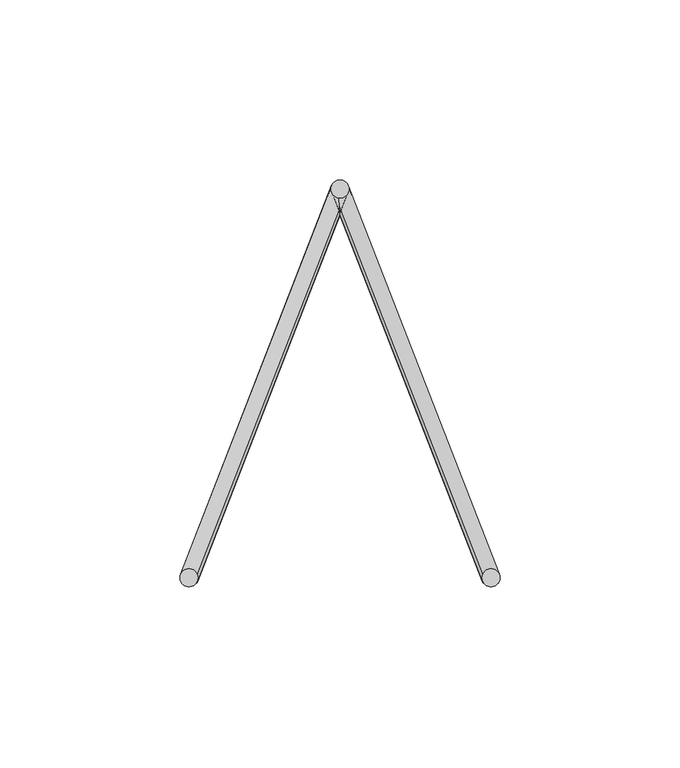
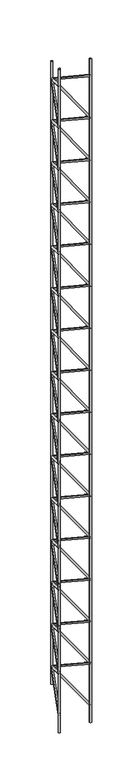
"""IFC4 building model written with IfcOpenShell, lengths in millimetres: proxy geometry, Pre-fab. (Vigota 1 - Pano 8)."""

from ifc_helpers import new_model, si_unit, point, frame, frame_2d, origin, origin_with_axes, origin_2d, place, context, project, spatial, circle_curve, trimmed, segment, composite_curve, outline, extrude, source, transform, mapped, element, save


def structural_framing_f61d2ecd(model_context):
    return source(origin(), model_context, "Body", "SweptSolid", [
        extrude(outline(composite_curve([segment(trimmed(circle_curve(origin_2d(), 2.5), [point((2.5, 0.0))], [point((-2.5, 0.0))], False, "CARTESIAN"), True, "CONTINUOUS"), segment(trimmed(circle_curve(origin_2d(), 2.5), [point((-2.5, 0.0))], [point((2.5, 0.0))], False, "CARTESIAN"), True, "CONTINUOUS")], self_intersect=False)), origin_with_axes(), (0.0, 0.0, 1.0), 1896.601886),
        extrude(outline(composite_curve([segment(trimmed(circle_curve(frame_2d((-42.0, 108.0)), 2.5), [point((-39.5, 108.0))], [point((-44.5, 108.0))], False, "CARTESIAN"), True, "CONTINUOUS"), segment(trimmed(circle_curve(frame_2d((-42.0, 108.0)), 2.5), [point((-44.5, 108.0))], [point((-39.5, 108.0))], False, "CARTESIAN"), True, "CONTINUOUS")], self_intersect=False)), frame((0.0, 0.0, 58.300943), z_axis=(0.0, 0.0, 1.0), x_axis=(1.0, 0.0, 0.0)), (0.0, 0.0, 1.0), 1780.0),
        extrude(outline(composite_curve([segment(trimmed(circle_curve(origin_2d(), 2.5), [point((2.5, 0.0))], [point((-2.5, 0.0))], False, "CARTESIAN"), True, "CONTINUOUS"), segment(trimmed(circle_curve(origin_2d(), 2.5), [point((-2.5, 0.0))], [point((2.5, 0.0))], False, "CARTESIAN"), True, "CONTINUOUS")], self_intersect=False)), frame((0.0, 0.0, 48.300943), z_axis=(-0.3218603428886276, 0.8276408817707567, 0.4598004898837537), x_axis=(0.8192319205108605, -3.936835275445103e-11, 0.5734623443750141)), (0.0, 0.0, 1.0), 130.491379),
        extrude(outline(composite_curve([segment(trimmed(circle_curve(origin_2d(), 2.5), [point((2.5, 0.0))], [point((-2.5, 0.0))], False, "CARTESIAN"), True, "CONTINUOUS"), segment(trimmed(circle_curve(origin_2d(), 2.5), [point((-2.5, 0.0))], [point((2.5, 0.0))], False, "CARTESIAN"), True, "CONTINUOUS")], self_intersect=False)), frame((-42.0, 108.0, 108.300943), z_axis=(0.3218603428886276, -0.8276408817707567, 0.4598004898837537), x_axis=(0.8192319205108605, -3.936835275445103e-11, -0.5734623443750141)), (0.0, 0.0, 1.0), 130.491379),
        extrude(outline(composite_curve([segment(trimmed(circle_curve(origin_2d(), 2.5), [point((2.5, 0.0))], [point((-2.5, 0.0))], False, "CARTESIAN"), True, "CONTINUOUS"), segment(trimmed(circle_curve(origin_2d(), 2.5), [point((-2.5, 0.0))], [point((2.5, 0.0))], False, "CARTESIAN"), True, "CONTINUOUS")], self_intersect=False)), frame((0.0, 0.0, 168.300943), z_axis=(-0.3218603428886276, 0.8276408817707567, 0.4598004898837537), x_axis=(0.8192319205108605, -3.936835275445103e-11, 0.5734623443750141)), (0.0, 0.0, 1.0), 130.491379),
        extrude(outline(composite_curve([segment(trimmed(circle_curve(origin_2d(), 2.5), [point((2.5, 0.0))], [point((-2.5, 0.0))], False, "CARTESIAN"), True, "CONTINUOUS"), segment(trimmed(circle_curve(origin_2d(), 2.5), [point((-2.5, 0.0))], [point((2.5, 0.0))], False, "CARTESIAN"), True, "CONTINUOUS")], self_intersect=False)), frame((-42.0, 108.0, 228.300943), z_axis=(0.3218603428886276, -0.8276408817707567, 0.4598004898837537), x_axis=(0.8192319205108605, -3.936835275445103e-11, -0.5734623443750141)), (0.0, 0.0, 1.0), 130.491379),
        extrude(outline(composite_curve([segment(trimmed(circle_curve(origin_2d(), 2.5), [point((2.5, 0.0))], [point((-2.5, 0.0))], False, "CARTESIAN"), True, "CONTINUOUS"), segment(trimmed(circle_curve(origin_2d(), 2.5), [point((-2.5, 0.0))], [point((2.5, 0.0))], False, "CARTESIAN"), True, "CONTINUOUS")], self_intersect=False)), frame((0.0, 0.0, 288.300943), z_axis=(-0.3218603428886276, 0.8276408817707567, 0.4598004898837537), x_axis=(0.8192319205108605, -3.936835275445103e-11, 0.5734623443750141)), (0.0, 0.0, 1.0), 130.491379),
        extrude(outline(composite_curve([segment(trimmed(circle_curve(origin_2d(), 2.5), [point((2.5, 0.0))], [point((-2.5, 0.0))], False, "CARTESIAN"), True, "CONTINUOUS"), segment(trimmed(circle_curve(origin_2d(), 2.5), [point((-2.5, 0.0))], [point((2.5, 0.0))], False, "CARTESIAN"), True, "CONTINUOUS")], self_intersect=False)), frame((-42.0, 108.0, 348.300943), z_axis=(0.3218603428886276, -0.8276408817707567, 0.4598004898837537), x_axis=(0.8192319205108605, -3.936835275445103e-11, -0.5734623443750141)), (0.0, 0.0, 1.0), 130.491379),
        extrude(outline(composite_curve([segment(trimmed(circle_curve(origin_2d(), 2.5), [point((2.5, 0.0))], [point((-2.5, 0.0))], False, "CARTESIAN"), True, "CONTINUOUS"), segment(trimmed(circle_curve(origin_2d(), 2.5), [point((-2.5, 0.0))], [point((2.5, 0.0))], False, "CARTESIAN"), True, "CONTINUOUS")], self_intersect=False)), frame((0.0, 0.0, 408.300943), z_axis=(-0.3218603428886276, 0.8276408817707567, 0.4598004898837537), x_axis=(0.8192319205108605, -3.936835275445103e-11, 0.5734623443750141)), (0.0, 0.0, 1.0), 130.491379),
        extrude(outline(composite_curve([segment(trimmed(circle_curve(origin_2d(), 2.5), [point((2.5, 0.0))], [point((-2.5, 0.0))], False, "CARTESIAN"), True, "CONTINUOUS"), segment(trimmed(circle_curve(origin_2d(), 2.5), [point((-2.5, 0.0))], [point((2.5, 0.0))], False, "CARTESIAN"), True, "CONTINUOUS")], self_intersect=False)), frame((-42.0, 108.0, 468.300943), z_axis=(0.3218603428886276, -0.8276408817707567, 0.4598004898837537), x_axis=(0.8192319205108605, -3.936835275445103e-11, -0.5734623443750141)), (0.0, 0.0, 1.0), 130.491379),
        extrude(outline(composite_curve([segment(trimmed(circle_curve(origin_2d(), 2.5), [point((2.5, 0.0))], [point((-2.5, 0.0))], False, "CARTESIAN"), True, "CONTINUOUS"), segment(trimmed(circle_curve(origin_2d(), 2.5), [point((-2.5, 0.0))], [point((2.5, 0.0))], False, "CARTESIAN"), True, "CONTINUOUS")], self_intersect=False)), frame((0.0, 0.0, 528.300943), z_axis=(-0.3218603428886276, 0.8276408817707567, 0.4598004898837537), x_axis=(0.8192319205108605, -3.936835275445103e-11, 0.5734623443750141)), (0.0, 0.0, 1.0), 130.491379),
        extrude(outline(composite_curve([segment(trimmed(circle_curve(origin_2d(), 2.5), [point((2.5, 0.0))], [point((-2.5, 0.0))], False, "CARTESIAN"), True, "CONTINUOUS"), segment(trimmed(circle_curve(origin_2d(), 2.5), [point((-2.5, 0.0))], [point((2.5, 0.0))], False, "CARTESIAN"), True, "CONTINUOUS")], self_intersect=False)), frame((-42.0, 108.0, 588.300943), z_axis=(0.3218603428886276, -0.8276408817707567, 0.4598004898837537), x_axis=(0.8192319205108605, -3.936835275445103e-11, -0.5734623443750141)), (0.0, 0.0, 1.0), 130.491379),
        extrude(outline(composite_curve([segment(trimmed(circle_curve(origin_2d(), 2.5), [point((2.5, 0.0))], [point((-2.5, 0.0))], False, "CARTESIAN"), True, "CONTINUOUS"), segment(trimmed(circle_curve(origin_2d(), 2.5), [point((-2.5, 0.0))], [point((2.5, 0.0))], False, "CARTESIAN"), True, "CONTINUOUS")], self_intersect=False)), frame((0.0, 0.0, 648.300943), z_axis=(-0.3218603428886276, 0.8276408817707567, 0.4598004898837537), x_axis=(0.8192319205108605, -3.936835275445103e-11, 0.5734623443750141)), (0.0, 0.0, 1.0), 130.491379),
        extrude(outline(composite_curve([segment(trimmed(circle_curve(origin_2d(), 2.5), [point((2.5, 0.0))], [point((-2.5, 0.0))], False, "CARTESIAN"), True, "CONTINUOUS"), segment(trimmed(circle_curve(origin_2d(), 2.5), [point((-2.5, 0.0))], [point((2.5, 0.0))], False, "CARTESIAN"), True, "CONTINUOUS")], self_intersect=False)), frame((-42.0, 108.0, 708.300943), z_axis=(0.3218603428886276, -0.8276408817707567, 0.4598004898837537), x_axis=(0.8192319205108605, -3.936835275445103e-11, -0.5734623443750141)), (0.0, 0.0, 1.0), 130.491379),
        extrude(outline(composite_curve([segment(trimmed(circle_curve(origin_2d(), 2.5), [point((2.5, 0.0))], [point((-2.5, 0.0))], False, "CARTESIAN"), True, "CONTINUOUS"), segment(trimmed(circle_curve(origin_2d(), 2.5), [point((-2.5, 0.0))], [point((2.5, 0.0))], False, "CARTESIAN"), True, "CONTINUOUS")], self_intersect=False)), frame((0.0, 0.0, 768.300943), z_axis=(-0.3218603428886276, 0.8276408817707567, 0.4598004898837537), x_axis=(0.8192319205108605, -3.936835275445103e-11, 0.5734623443750141)), (0.0, 0.0, 1.0), 130.491379),
        extrude(outline(composite_curve([segment(trimmed(circle_curve(origin_2d(), 2.5), [point((2.5, 0.0))], [point((-2.5, 0.0))], False, "CARTESIAN"), True, "CONTINUOUS"), segment(trimmed(circle_curve(origin_2d(), 2.5), [point((-2.5, 0.0))], [point((2.5, 0.0))], False, "CARTESIAN"), True, "CONTINUOUS")], self_intersect=False)), frame((-42.0, 108.0, 828.300943), z_axis=(0.3218603428886276, -0.8276408817707567, 0.4598004898837537), x_axis=(0.8192319205108605, -3.936835275445103e-11, -0.5734623443750141)), (0.0, 0.0, 1.0), 130.491379),
        extrude(outline(composite_curve([segment(trimmed(circle_curve(origin_2d(), 2.5), [point((2.5, 0.0))], [point((-2.5, 0.0))], False, "CARTESIAN"), True, "CONTINUOUS"), segment(trimmed(circle_curve(origin_2d(), 2.5), [point((-2.5, 0.0))], [point((2.5, 0.0))], False, "CARTESIAN"), True, "CONTINUOUS")], self_intersect=False)), frame((0.0, 0.0, 888.300943), z_axis=(-0.3218603428886276, 0.8276408817707567, 0.4598004898837537), x_axis=(0.8192319205108605, -3.936835275445103e-11, 0.5734623443750141)), (0.0, 0.0, 1.0), 130.491379),
        extrude(outline(composite_curve([segment(trimmed(circle_curve(origin_2d(), 2.5), [point((2.5, 0.0))], [point((-2.5, 0.0))], False, "CARTESIAN"), True, "CONTINUOUS"), segment(trimmed(circle_curve(origin_2d(), 2.5), [point((-2.5, 0.0))], [point((2.5, 0.0))], False, "CARTESIAN"), True, "CONTINUOUS")], self_intersect=False)), frame((-42.0, 108.0, 948.300943), z_axis=(0.3218603428886276, -0.8276408817707567, 0.4598004898837537), x_axis=(0.8192319205108605, -3.936835275445103e-11, -0.5734623443750141)), (0.0, 0.0, 1.0), 130.491379),
        extrude(outline(composite_curve([segment(trimmed(circle_curve(origin_2d(), 2.5), [point((2.5, 0.0))], [point((-2.5, 0.0))], False, "CARTESIAN"), True, "CONTINUOUS"), segment(trimmed(circle_curve(origin_2d(), 2.5), [point((-2.5, 0.0))], [point((2.5, 0.0))], False, "CARTESIAN"), True, "CONTINUOUS")], self_intersect=False)), frame((0.0, 0.0, 1008.300943), z_axis=(-0.3218603428886276, 0.8276408817707567, 0.4598004898837537), x_axis=(0.8192319205108605, -3.936835275445103e-11, 0.5734623443750141)), (0.0, 0.0, 1.0), 130.491379),
        extrude(outline(composite_curve([segment(trimmed(circle_curve(origin_2d(), 2.5), [point((2.5, 0.0))], [point((-2.5, 0.0))], False, "CARTESIAN"), True, "CONTINUOUS"), segment(trimmed(circle_curve(origin_2d(), 2.5), [point((-2.5, 0.0))], [point((2.5, 0.0))], False, "CARTESIAN"), True, "CONTINUOUS")], self_intersect=False)), frame((-42.0, 108.0, 1068.300943), z_axis=(0.3218603428886276, -0.8276408817707567, 0.4598004898837537), x_axis=(0.8192319205108605, -3.936835275445103e-11, -0.5734623443750141)), (0.0, 0.0, 1.0), 130.491379),
        extrude(outline(composite_curve([segment(trimmed(circle_curve(origin_2d(), 2.5), [point((2.5, 0.0))], [point((-2.5, 0.0))], False, "CARTESIAN"), True, "CONTINUOUS"), segment(trimmed(circle_curve(origin_2d(), 2.5), [point((-2.5, 0.0))], [point((2.5, 0.0))], False, "CARTESIAN"), True, "CONTINUOUS")], self_intersect=False)), frame((0.0, 0.0, 1128.300943), z_axis=(-0.3218603428886276, 0.8276408817707567, 0.4598004898837537), x_axis=(0.8192319205108605, -3.936835275445103e-11, 0.5734623443750141)), (0.0, 0.0, 1.0), 130.491379),
        extrude(outline(composite_curve([segment(trimmed(circle_curve(origin_2d(), 2.5), [point((2.5, 0.0))], [point((-2.5, 0.0))], False, "CARTESIAN"), True, "CONTINUOUS"), segment(trimmed(circle_curve(origin_2d(), 2.5), [point((-2.5, 0.0))], [point((2.5, 0.0))], False, "CARTESIAN"), True, "CONTINUOUS")], self_intersect=False)), frame((-42.0, 108.0, 1188.300943), z_axis=(0.3218603428886276, -0.8276408817707567, 0.4598004898837537), x_axis=(0.8192319205108605, -3.936835275445103e-11, -0.5734623443750141)), (0.0, 0.0, 1.0), 130.491379),
        extrude(outline(composite_curve([segment(trimmed(circle_curve(origin_2d(), 2.5), [point((2.5, 0.0))], [point((-2.5, 0.0))], False, "CARTESIAN"), True, "CONTINUOUS"), segment(trimmed(circle_curve(origin_2d(), 2.5), [point((-2.5, 0.0))], [point((2.5, 0.0))], False, "CARTESIAN"), True, "CONTINUOUS")], self_intersect=False)), frame((0.0, 0.0, 1248.300943), z_axis=(-0.3218603428886276, 0.8276408817707567, 0.4598004898837537), x_axis=(0.8192319205108605, -3.936835275445103e-11, 0.5734623443750141)), (0.0, 0.0, 1.0), 130.491379),
        extrude(outline(composite_curve([segment(trimmed(circle_curve(origin_2d(), 2.5), [point((2.5, 0.0))], [point((-2.5, 0.0))], False, "CARTESIAN"), True, "CONTINUOUS"), segment(trimmed(circle_curve(origin_2d(), 2.5), [point((-2.5, 0.0))], [point((2.5, 0.0))], False, "CARTESIAN"), True, "CONTINUOUS")], self_intersect=False)), frame((-42.0, 108.0, 1308.300943), z_axis=(0.3218603428886276, -0.8276408817707567, 0.4598004898837537), x_axis=(0.8192319205108605, -3.936835275445103e-11, -0.5734623443750141)), (0.0, 0.0, 1.0), 130.491379),
        extrude(outline(composite_curve([segment(trimmed(circle_curve(origin_2d(), 2.5), [point((2.5, 0.0))], [point((-2.5, 0.0))], False, "CARTESIAN"), True, "CONTINUOUS"), segment(trimmed(circle_curve(origin_2d(), 2.5), [point((-2.5, 0.0))], [point((2.5, 0.0))], False, "CARTESIAN"), True, "CONTINUOUS")], self_intersect=False)), frame((0.0, 0.0, 1368.300943), z_axis=(-0.3218603428886276, 0.8276408817707567, 0.4598004898837537), x_axis=(0.8192319205108605, -3.936835275445103e-11, 0.5734623443750141)), (0.0, 0.0, 1.0), 130.491379),
        extrude(outline(composite_curve([segment(trimmed(circle_curve(origin_2d(), 2.5), [point((2.5, 0.0))], [point((-2.5, 0.0))], False, "CARTESIAN"), True, "CONTINUOUS"), segment(trimmed(circle_curve(origin_2d(), 2.5), [point((-2.5, 0.0))], [point((2.5, 0.0))], False, "CARTESIAN"), True, "CONTINUOUS")], self_intersect=False)), frame((-42.0, 108.0, 1428.300943), z_axis=(0.3218603428886276, -0.8276408817707567, 0.4598004898837537), x_axis=(0.8192319205108605, -3.936835275445103e-11, -0.5734623443750141)), (0.0, 0.0, 1.0), 130.491379),
        extrude(outline(composite_curve([segment(trimmed(circle_curve(origin_2d(), 2.5), [point((2.5, 0.0))], [point((-2.5, 0.0))], False, "CARTESIAN"), True, "CONTINUOUS"), segment(trimmed(circle_curve(origin_2d(), 2.5), [point((-2.5, 0.0))], [point((2.5, 0.0))], False, "CARTESIAN"), True, "CONTINUOUS")], self_intersect=False)), frame((0.0, 0.0, 1488.300943), z_axis=(-0.3218603428886276, 0.8276408817707567, 0.4598004898837537), x_axis=(0.8192319205108605, -3.936835275445103e-11, 0.5734623443750141)), (0.0, 0.0, 1.0), 130.491379),
        extrude(outline(composite_curve([segment(trimmed(circle_curve(origin_2d(), 2.5), [point((2.5, 0.0))], [point((-2.5, 0.0))], False, "CARTESIAN"), True, "CONTINUOUS"), segment(trimmed(circle_curve(origin_2d(), 2.5), [point((-2.5, 0.0))], [point((2.5, 0.0))], False, "CARTESIAN"), True, "CONTINUOUS")], self_intersect=False)), frame((-42.0, 108.0, 1548.300943), z_axis=(0.3218603428886276, -0.8276408817707567, 0.4598004898837537), x_axis=(0.8192319205108605, -3.936835275445103e-11, -0.5734623443750141)), (0.0, 0.0, 1.0), 130.491379),
        extrude(outline(composite_curve([segment(trimmed(circle_curve(origin_2d(), 2.5), [point((2.5, 0.0))], [point((-2.5, 0.0))], False, "CARTESIAN"), True, "CONTINUOUS"), segment(trimmed(circle_curve(origin_2d(), 2.5), [point((-2.5, 0.0))], [point((2.5, 0.0))], False, "CARTESIAN"), True, "CONTINUOUS")], self_intersect=False)), frame((0.0, 0.0, 1608.300943), z_axis=(-0.3218603428886276, 0.8276408817707567, 0.4598004898837537), x_axis=(0.8192319205108605, -3.936835275445103e-11, 0.5734623443750141)), (0.0, 0.0, 1.0), 130.491379),
        extrude(outline(composite_curve([segment(trimmed(circle_curve(origin_2d(), 2.5), [point((2.5, 0.0))], [point((-2.5, 0.0))], False, "CARTESIAN"), True, "CONTINUOUS"), segment(trimmed(circle_curve(origin_2d(), 2.5), [point((-2.5, 0.0))], [point((2.5, 0.0))], False, "CARTESIAN"), True, "CONTINUOUS")], self_intersect=False)), frame((-42.0, 108.0, 1668.300943), z_axis=(0.3218603428886276, -0.8276408817707567, 0.4598004898837537), x_axis=(0.8192319205108605, -3.936835275445103e-11, -0.5734623443750141)), (0.0, 0.0, 1.0), 130.491379),
        extrude(outline(composite_curve([segment(trimmed(circle_curve(origin_2d(), 2.5), [point((2.5, 0.0))], [point((-2.5, 0.0))], False, "CARTESIAN"), True, "CONTINUOUS"), segment(trimmed(circle_curve(origin_2d(), 2.5), [point((-2.5, 0.0))], [point((2.5, 0.0))], False, "CARTESIAN"), True, "CONTINUOUS")], self_intersect=False)), frame((0.0, 0.0, 1728.300943), z_axis=(-0.3218603428886276, 0.8276408817707567, 0.4598004898837537), x_axis=(0.8192319205108605, -3.936835275445103e-11, 0.5734623443750141)), (0.0, 0.0, 1.0), 130.491379),
        extrude(outline(composite_curve([segment(trimmed(circle_curve(origin_2d(), 2.5), [point((2.5, 0.0))], [point((-2.5, 0.0))], False, "CARTESIAN"), True, "CONTINUOUS"), segment(trimmed(circle_curve(origin_2d(), 2.5), [point((-2.5, 0.0))], [point((2.5, 0.0))], False, "CARTESIAN"), True, "CONTINUOUS")], self_intersect=False)), frame((-42.0, 108.0, 1788.300943), z_axis=(0.3218603428886276, -0.8276408817707567, 0.4598004898837537), x_axis=(0.8192319205108605, -3.936835275445103e-11, -0.5734623443750141)), (0.0, 0.0, 1.0), 130.491379),
        extrude(outline(composite_curve([segment(trimmed(circle_curve(frame_2d((-84.0, 0.0)), 2.5), [point((-81.5, 0.0))], [point((-86.5, 0.0))], False, "CARTESIAN"), True, "CONTINUOUS"), segment(trimmed(circle_curve(frame_2d((-84.0, 0.0)), 2.5), [point((-86.5, 0.0))], [point((-81.5, 0.0))], False, "CARTESIAN"), True, "CONTINUOUS")], self_intersect=False)), origin_with_axes(), (0.0, 0.0, 1.0), 1896.601886),
        extrude(outline(composite_curve([segment(trimmed(circle_curve(origin_2d(), 2.5), [point((2.5, 0.0))], [point((-2.5, 0.0))], False, "CARTESIAN"), True, "CONTINUOUS"), segment(trimmed(circle_curve(origin_2d(), 2.5), [point((-2.5, 0.0))], [point((2.5, 0.0))], False, "CARTESIAN"), True, "CONTINUOUS")], self_intersect=False)), frame((-84.0, 0.0, 48.300943), z_axis=(0.3218603428886276, 0.8276408817707567, 0.4598004898837537), x_axis=(0.8192319205108605, 3.936835275445103e-11, -0.5734623443750141)), (0.0, 0.0, 1.0), 130.491379),
        extrude(outline(composite_curve([segment(trimmed(circle_curve(origin_2d(), 2.5), [point((2.5, 0.0))], [point((-2.5, 0.0))], False, "CARTESIAN"), True, "CONTINUOUS"), segment(trimmed(circle_curve(origin_2d(), 2.5), [point((-2.5, 0.0))], [point((2.5, 0.0))], False, "CARTESIAN"), True, "CONTINUOUS")], self_intersect=False)), frame((-42.0, 108.0, 108.300943), z_axis=(-0.3218603428886276, -0.8276408817707567, 0.4598004898837537), x_axis=(0.8192319205108605, 3.936835275445103e-11, 0.5734623443750141)), (0.0, 0.0, 1.0), 130.491379),
        extrude(outline(composite_curve([segment(trimmed(circle_curve(origin_2d(), 2.5), [point((2.5, 0.0))], [point((-2.5, 0.0))], False, "CARTESIAN"), True, "CONTINUOUS"), segment(trimmed(circle_curve(origin_2d(), 2.5), [point((-2.5, 0.0))], [point((2.5, 0.0))], False, "CARTESIAN"), True, "CONTINUOUS")], self_intersect=False)), frame((-84.0, 0.0, 168.300943), z_axis=(0.3218603428886276, 0.8276408817707567, 0.4598004898837537), x_axis=(0.8192319205108605, 3.936835275445103e-11, -0.5734623443750141)), (0.0, 0.0, 1.0), 130.491379),
        extrude(outline(composite_curve([segment(trimmed(circle_curve(origin_2d(), 2.5), [point((2.5, 0.0))], [point((-2.5, 0.0))], False, "CARTESIAN"), True, "CONTINUOUS"), segment(trimmed(circle_curve(origin_2d(), 2.5), [point((-2.5, 0.0))], [point((2.5, 0.0))], False, "CARTESIAN"), True, "CONTINUOUS")], self_intersect=False)), frame((-42.0, 108.0, 228.300943), z_axis=(-0.3218603428886276, -0.8276408817707567, 0.4598004898837537), x_axis=(0.8192319205108605, 3.936835275445103e-11, 0.5734623443750141)), (0.0, 0.0, 1.0), 130.491379),
        extrude(outline(composite_curve([segment(trimmed(circle_curve(origin_2d(), 2.5), [point((2.5, 0.0))], [point((-2.5, 0.0))], False, "CARTESIAN"), True, "CONTINUOUS"), segment(trimmed(circle_curve(origin_2d(), 2.5), [point((-2.5, 0.0))], [point((2.5, 0.0))], False, "CARTESIAN"), True, "CONTINUOUS")], self_intersect=False)), frame((-84.0, 0.0, 288.300943), z_axis=(0.3218603428886276, 0.8276408817707567, 0.4598004898837537), x_axis=(0.8192319205108605, 3.936835275445103e-11, -0.5734623443750141)), (0.0, 0.0, 1.0), 130.491379),
        extrude(outline(composite_curve([segment(trimmed(circle_curve(origin_2d(), 2.5), [point((2.5, 0.0))], [point((-2.5, 0.0))], False, "CARTESIAN"), True, "CONTINUOUS"), segment(trimmed(circle_curve(origin_2d(), 2.5), [point((-2.5, 0.0))], [point((2.5, 0.0))], False, "CARTESIAN"), True, "CONTINUOUS")], self_intersect=False)), frame((-42.0, 108.0, 348.300943), z_axis=(-0.3218603428886276, -0.8276408817707567, 0.4598004898837537), x_axis=(0.8192319205108605, 3.936835275445103e-11, 0.5734623443750141)), (0.0, 0.0, 1.0), 130.491379),
        extrude(outline(composite_curve([segment(trimmed(circle_curve(origin_2d(), 2.5), [point((2.5, 0.0))], [point((-2.5, 0.0))], False, "CARTESIAN"), True, "CONTINUOUS"), segment(trimmed(circle_curve(origin_2d(), 2.5), [point((-2.5, 0.0))], [point((2.5, 0.0))], False, "CARTESIAN"), True, "CONTINUOUS")], self_intersect=False)), frame((-84.0, 0.0, 408.300943), z_axis=(0.3218603428886276, 0.8276408817707567, 0.4598004898837537), x_axis=(0.8192319205108605, 3.936835275445103e-11, -0.5734623443750141)), (0.0, 0.0, 1.0), 130.491379),
        extrude(outline(composite_curve([segment(trimmed(circle_curve(origin_2d(), 2.5), [point((2.5, 0.0))], [point((-2.5, 0.0))], False, "CARTESIAN"), True, "CONTINUOUS"), segment(trimmed(circle_curve(origin_2d(), 2.5), [point((-2.5, 0.0))], [point((2.5, 0.0))], False, "CARTESIAN"), True, "CONTINUOUS")], self_intersect=False)), frame((-42.0, 108.0, 468.300943), z_axis=(-0.3218603428886276, -0.8276408817707567, 0.4598004898837537), x_axis=(0.8192319205108605, 3.936835275445103e-11, 0.5734623443750141)), (0.0, 0.0, 1.0), 130.491379),
        extrude(outline(composite_curve([segment(trimmed(circle_curve(origin_2d(), 2.5), [point((2.5, 0.0))], [point((-2.5, 0.0))], False, "CARTESIAN"), True, "CONTINUOUS"), segment(trimmed(circle_curve(origin_2d(), 2.5), [point((-2.5, 0.0))], [point((2.5, 0.0))], False, "CARTESIAN"), True, "CONTINUOUS")], self_intersect=False)), frame((-84.0, 0.0, 528.300943), z_axis=(0.3218603428886276, 0.8276408817707567, 0.4598004898837537), x_axis=(0.8192319205108605, 3.936835275445103e-11, -0.5734623443750141)), (0.0, 0.0, 1.0), 130.491379),
        extrude(outline(composite_curve([segment(trimmed(circle_curve(origin_2d(), 2.5), [point((2.5, 0.0))], [point((-2.5, 0.0))], False, "CARTESIAN"), True, "CONTINUOUS"), segment(trimmed(circle_curve(origin_2d(), 2.5), [point((-2.5, 0.0))], [point((2.5, 0.0))], False, "CARTESIAN"), True, "CONTINUOUS")], self_intersect=False)), frame((-42.0, 108.0, 588.300943), z_axis=(-0.3218603428886276, -0.8276408817707567, 0.4598004898837537), x_axis=(0.8192319205108605, 3.936835275445103e-11, 0.5734623443750141)), (0.0, 0.0, 1.0), 130.491379),
        extrude(outline(composite_curve([segment(trimmed(circle_curve(origin_2d(), 2.5), [point((2.5, 0.0))], [point((-2.5, 0.0))], False, "CARTESIAN"), True, "CONTINUOUS"), segment(trimmed(circle_curve(origin_2d(), 2.5), [point((-2.5, 0.0))], [point((2.5, 0.0))], False, "CARTESIAN"), True, "CONTINUOUS")], self_intersect=False)), frame((-84.0, 0.0, 648.300943), z_axis=(0.3218603428886276, 0.8276408817707567, 0.4598004898837537), x_axis=(0.8192319205108605, 3.936835275445103e-11, -0.5734623443750141)), (0.0, 0.0, 1.0), 130.491379),
        extrude(outline(composite_curve([segment(trimmed(circle_curve(origin_2d(), 2.5), [point((2.5, 0.0))], [point((-2.5, 0.0))], False, "CARTESIAN"), True, "CONTINUOUS"), segment(trimmed(circle_curve(origin_2d(), 2.5), [point((-2.5, 0.0))], [point((2.5, 0.0))], False, "CARTESIAN"), True, "CONTINUOUS")], self_intersect=False)), frame((-42.0, 108.0, 708.300943), z_axis=(-0.3218603428886276, -0.8276408817707567, 0.4598004898837537), x_axis=(0.8192319205108605, 3.936835275445103e-11, 0.5734623443750141)), (0.0, 0.0, 1.0), 130.491379),
        extrude(outline(composite_curve([segment(trimmed(circle_curve(origin_2d(), 2.5), [point((2.5, 0.0))], [point((-2.5, 0.0))], False, "CARTESIAN"), True, "CONTINUOUS"), segment(trimmed(circle_curve(origin_2d(), 2.5), [point((-2.5, 0.0))], [point((2.5, 0.0))], False, "CARTESIAN"), True, "CONTINUOUS")], self_intersect=False)), frame((-84.0, 0.0, 768.300943), z_axis=(0.3218603428886276, 0.8276408817707567, 0.4598004898837537), x_axis=(0.8192319205108605, 3.936835275445103e-11, -0.5734623443750141)), (0.0, 0.0, 1.0), 130.491379),
        extrude(outline(composite_curve([segment(trimmed(circle_curve(origin_2d(), 2.5), [point((2.5, 0.0))], [point((-2.5, 0.0))], False, "CARTESIAN"), True, "CONTINUOUS"), segment(trimmed(circle_curve(origin_2d(), 2.5), [point((-2.5, 0.0))], [point((2.5, 0.0))], False, "CARTESIAN"), True, "CONTINUOUS")], self_intersect=False)), frame((-42.0, 108.0, 828.300943), z_axis=(-0.3218603428886276, -0.8276408817707567, 0.4598004898837537), x_axis=(0.8192319205108605, 3.936835275445103e-11, 0.5734623443750141)), (0.0, 0.0, 1.0), 130.491379),
        extrude(outline(composite_curve([segment(trimmed(circle_curve(origin_2d(), 2.5), [point((2.5, 0.0))], [point((-2.5, 0.0))], False, "CARTESIAN"), True, "CONTINUOUS"), segment(trimmed(circle_curve(origin_2d(), 2.5), [point((-2.5, 0.0))], [point((2.5, 0.0))], False, "CARTESIAN"), True, "CONTINUOUS")], self_intersect=False)), frame((-84.0, 0.0, 888.300943), z_axis=(0.3218603428886276, 0.8276408817707567, 0.4598004898837537), x_axis=(0.8192319205108605, 3.936835275445103e-11, -0.5734623443750141)), (0.0, 0.0, 1.0), 130.491379),
        extrude(outline(composite_curve([segment(trimmed(circle_curve(origin_2d(), 2.5), [point((2.5, 0.0))], [point((-2.5, 0.0))], False, "CARTESIAN"), True, "CONTINUOUS"), segment(trimmed(circle_curve(origin_2d(), 2.5), [point((-2.5, 0.0))], [point((2.5, 0.0))], False, "CARTESIAN"), True, "CONTINUOUS")], self_intersect=False)), frame((-42.0, 108.0, 948.300943), z_axis=(-0.3218603428886276, -0.8276408817707567, 0.4598004898837537), x_axis=(0.8192319205108605, 3.936835275445103e-11, 0.5734623443750141)), (0.0, 0.0, 1.0), 130.491379),
        extrude(outline(composite_curve([segment(trimmed(circle_curve(origin_2d(), 2.5), [point((2.5, 0.0))], [point((-2.5, 0.0))], False, "CARTESIAN"), True, "CONTINUOUS"), segment(trimmed(circle_curve(origin_2d(), 2.5), [point((-2.5, 0.0))], [point((2.5, 0.0))], False, "CARTESIAN"), True, "CONTINUOUS")], self_intersect=False)), frame((-84.0, 0.0, 1008.300943), z_axis=(0.3218603428886276, 0.8276408817707567, 0.4598004898837537), x_axis=(0.8192319205108605, 3.936835275445103e-11, -0.5734623443750141)), (0.0, 0.0, 1.0), 130.491379),
        extrude(outline(composite_curve([segment(trimmed(circle_curve(origin_2d(), 2.5), [point((2.5, 0.0))], [point((-2.5, 0.0))], False, "CARTESIAN"), True, "CONTINUOUS"), segment(trimmed(circle_curve(origin_2d(), 2.5), [point((-2.5, 0.0))], [point((2.5, 0.0))], False, "CARTESIAN"), True, "CONTINUOUS")], self_intersect=False)), frame((-42.0, 108.0, 1068.300943), z_axis=(-0.3218603428886276, -0.8276408817707567, 0.4598004898837537), x_axis=(0.8192319205108605, 3.936835275445103e-11, 0.5734623443750141)), (0.0, 0.0, 1.0), 130.491379),
        extrude(outline(composite_curve([segment(trimmed(circle_curve(origin_2d(), 2.5), [point((2.5, 0.0))], [point((-2.5, 0.0))], False, "CARTESIAN"), True, "CONTINUOUS"), segment(trimmed(circle_curve(origin_2d(), 2.5), [point((-2.5, 0.0))], [point((2.5, 0.0))], False, "CARTESIAN"), True, "CONTINUOUS")], self_intersect=False)), frame((-84.0, 0.0, 1128.300943), z_axis=(0.3218603428886276, 0.8276408817707567, 0.4598004898837537), x_axis=(0.8192319205108605, 3.936835275445103e-11, -0.5734623443750141)), (0.0, 0.0, 1.0), 130.491379),
        extrude(outline(composite_curve([segment(trimmed(circle_curve(origin_2d(), 2.5), [point((2.5, 0.0))], [point((-2.5, 0.0))], False, "CARTESIAN"), True, "CONTINUOUS"), segment(trimmed(circle_curve(origin_2d(), 2.5), [point((-2.5, 0.0))], [point((2.5, 0.0))], False, "CARTESIAN"), True, "CONTINUOUS")], self_intersect=False)), frame((-42.0, 108.0, 1188.300943), z_axis=(-0.3218603428886276, -0.8276408817707567, 0.4598004898837537), x_axis=(0.8192319205108605, 3.936835275445103e-11, 0.5734623443750141)), (0.0, 0.0, 1.0), 130.491379),
        extrude(outline(composite_curve([segment(trimmed(circle_curve(origin_2d(), 2.5), [point((2.5, 0.0))], [point((-2.5, 0.0))], False, "CARTESIAN"), True, "CONTINUOUS"), segment(trimmed(circle_curve(origin_2d(), 2.5), [point((-2.5, 0.0))], [point((2.5, 0.0))], False, "CARTESIAN"), True, "CONTINUOUS")], self_intersect=False)), frame((-84.0, 0.0, 1248.300943), z_axis=(0.3218603428886276, 0.8276408817707567, 0.4598004898837537), x_axis=(0.8192319205108605, 3.936835275445103e-11, -0.5734623443750141)), (0.0, 0.0, 1.0), 130.491379),
        extrude(outline(composite_curve([segment(trimmed(circle_curve(origin_2d(), 2.5), [point((2.5, 0.0))], [point((-2.5, 0.0))], False, "CARTESIAN"), True, "CONTINUOUS"), segment(trimmed(circle_curve(origin_2d(), 2.5), [point((-2.5, 0.0))], [point((2.5, 0.0))], False, "CARTESIAN"), True, "CONTINUOUS")], self_intersect=False)), frame((-42.0, 108.0, 1308.300943), z_axis=(-0.3218603428886276, -0.8276408817707567, 0.4598004898837537), x_axis=(0.8192319205108605, 3.936835275445103e-11, 0.5734623443750141)), (0.0, 0.0, 1.0), 130.491379),
        extrude(outline(composite_curve([segment(trimmed(circle_curve(origin_2d(), 2.5), [point((2.5, 0.0))], [point((-2.5, 0.0))], False, "CARTESIAN"), True, "CONTINUOUS"), segment(trimmed(circle_curve(origin_2d(), 2.5), [point((-2.5, 0.0))], [point((2.5, 0.0))], False, "CARTESIAN"), True, "CONTINUOUS")], self_intersect=False)), frame((-84.0, 0.0, 1368.300943), z_axis=(0.3218603428886276, 0.8276408817707567, 0.4598004898837537), x_axis=(0.8192319205108605, 3.936835275445103e-11, -0.5734623443750141)), (0.0, 0.0, 1.0), 130.491379),
        extrude(outline(composite_curve([segment(trimmed(circle_curve(origin_2d(), 2.5), [point((2.5, 0.0))], [point((-2.5, 0.0))], False, "CARTESIAN"), True, "CONTINUOUS"), segment(trimmed(circle_curve(origin_2d(), 2.5), [point((-2.5, 0.0))], [point((2.5, 0.0))], False, "CARTESIAN"), True, "CONTINUOUS")], self_intersect=False)), frame((-42.0, 108.0, 1428.300943), z_axis=(-0.3218603428886276, -0.8276408817707567, 0.4598004898837537), x_axis=(0.8192319205108605, 3.936835275445103e-11, 0.5734623443750141)), (0.0, 0.0, 1.0), 130.491379),
        extrude(outline(composite_curve([segment(trimmed(circle_curve(origin_2d(), 2.5), [point((2.5, 0.0))], [point((-2.5, 0.0))], False, "CARTESIAN"), True, "CONTINUOUS"), segment(trimmed(circle_curve(origin_2d(), 2.5), [point((-2.5, 0.0))], [point((2.5, 0.0))], False, "CARTESIAN"), True, "CONTINUOUS")], self_intersect=False)), frame((-84.0, 0.0, 1488.300943), z_axis=(0.3218603428886276, 0.8276408817707567, 0.4598004898837537), x_axis=(0.8192319205108605, 3.936835275445103e-11, -0.5734623443750141)), (0.0, 0.0, 1.0), 130.491379),
        extrude(outline(composite_curve([segment(trimmed(circle_curve(origin_2d(), 2.5), [point((2.5, 0.0))], [point((-2.5, 0.0))], False, "CARTESIAN"), True, "CONTINUOUS"), segment(trimmed(circle_curve(origin_2d(), 2.5), [point((-2.5, 0.0))], [point((2.5, 0.0))], False, "CARTESIAN"), True, "CONTINUOUS")], self_intersect=False)), frame((-42.0, 108.0, 1548.300943), z_axis=(-0.3218603428886276, -0.8276408817707567, 0.4598004898837537), x_axis=(0.8192319205108605, 3.936835275445103e-11, 0.5734623443750141)), (0.0, 0.0, 1.0), 130.491379),
        extrude(outline(composite_curve([segment(trimmed(circle_curve(origin_2d(), 2.5), [point((2.5, 0.0))], [point((-2.5, 0.0))], False, "CARTESIAN"), True, "CONTINUOUS"), segment(trimmed(circle_curve(origin_2d(), 2.5), [point((-2.5, 0.0))], [point((2.5, 0.0))], False, "CARTESIAN"), True, "CONTINUOUS")], self_intersect=False)), frame((-84.0, 0.0, 1608.300943), z_axis=(0.3218603428886276, 0.8276408817707567, 0.4598004898837537), x_axis=(0.8192319205108605, 3.936835275445103e-11, -0.5734623443750141)), (0.0, 0.0, 1.0), 130.491379),
        extrude(outline(composite_curve([segment(trimmed(circle_curve(origin_2d(), 2.5), [point((2.5, 0.0))], [point((-2.5, 0.0))], False, "CARTESIAN"), True, "CONTINUOUS"), segment(trimmed(circle_curve(origin_2d(), 2.5), [point((-2.5, 0.0))], [point((2.5, 0.0))], False, "CARTESIAN"), True, "CONTINUOUS")], self_intersect=False)), frame((-42.0, 108.0, 1668.300943), z_axis=(-0.3218603428886276, -0.8276408817707567, 0.4598004898837537), x_axis=(0.8192319205108605, 3.936835275445103e-11, 0.5734623443750141)), (0.0, 0.0, 1.0), 130.491379),
        extrude(outline(composite_curve([segment(trimmed(circle_curve(origin_2d(), 2.5), [point((2.5, 0.0))], [point((-2.5, 0.0))], False, "CARTESIAN"), True, "CONTINUOUS"), segment(trimmed(circle_curve(origin_2d(), 2.5), [point((-2.5, 0.0))], [point((2.5, 0.0))], False, "CARTESIAN"), True, "CONTINUOUS")], self_intersect=False)), frame((-84.0, 0.0, 1728.300943), z_axis=(0.3218603428886276, 0.8276408817707567, 0.4598004898837537), x_axis=(0.8192319205108605, 3.936835275445103e-11, -0.5734623443750141)), (0.0, 0.0, 1.0), 130.491379),
        extrude(outline(composite_curve([segment(trimmed(circle_curve(origin_2d(), 2.5), [point((2.5, 0.0))], [point((-2.5, 0.0))], False, "CARTESIAN"), True, "CONTINUOUS"), segment(trimmed(circle_curve(origin_2d(), 2.5), [point((-2.5, 0.0))], [point((2.5, 0.0))], False, "CARTESIAN"), True, "CONTINUOUS")], self_intersect=False)), frame((-42.0, 108.0, 1788.300943), z_axis=(-0.3218603428886276, -0.8276408817707567, 0.4598004898837537), x_axis=(0.8192319205108605, 3.936835275445103e-11, 0.5734623443750141)), (0.0, 0.0, 1.0), 130.491379),
    ])


if __name__ == "__main__":
    model = new_model("IFC4")
    model_context = context("Model", 3, world=origin())
    ifc_project = project(units=[si_unit("LENGTHUNIT", "METRE", prefix="MILLI")], contexts=[model_context])
    site = spatial("IfcSite", under=ifc_project)
    building = spatial("IfcBuilding", under=site)
    placement = place(None, origin())
    structural_framing_shape = structural_framing_f61d2ecd(model_context)
    element("IfcBuildingElementProxy", 1, Name="Pre-fab. (Vigota 1 - Pano 8)", ObjectType="Pre-fab. (Vigota 1 - Pano 8)", at=placement, inside=building, context=model_context, shape_type="MappedRepresentation", body=[
        mapped(structural_framing_shape, transform((0.0, 0.0, 0.0), x_axis=(1.0, 0.0, 0.0), y_axis=(0.0, 1.0, 0.0), z_axis=(0.0, 0.0, 1.0))),
    ])
    save(model, "model.ifc")

# Revit data of these elements
# Element 1 (IfcBuildingElementProxy, "Pre-fab. (Vigota 1 - Pano 8)")
#   Materials on its faces: "Aço"
# Materials
#   "Aço": class "Metal", colour RGB 120 120 120, transparency 0, Description = "Aço estrutural A36 grau, ASTM B, acabamento laminado", Cost = 0
